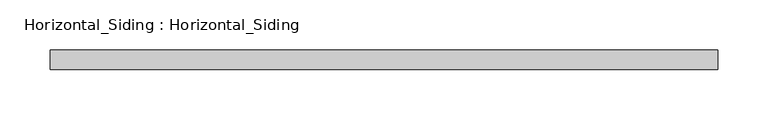
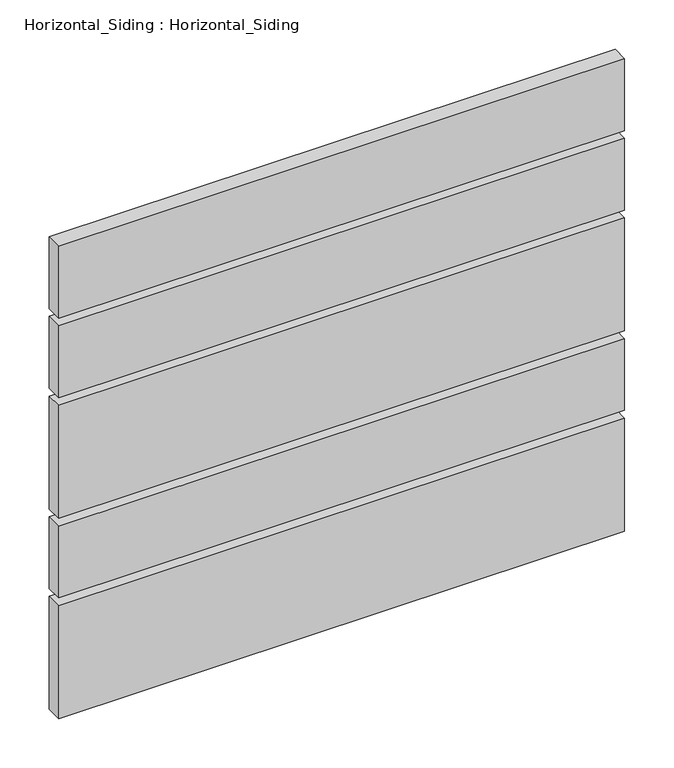
"""IFC4 building model written with IfcOpenShell, lengths in millimetres: plate geometry, Horizontal_Siding : Horizontal_Siding."""

import ifcopenshell
import ifcopenshell.guid

model = None  # the IFC model being written
_history = None  # IfcOwnerHistory: only IFC2X3 demands one
_inside = {}  # id of a spatial element -> (the spatial element, [elements in it])
_under = {}  # id of a project, library or spatial element -> (it, [spatial elements below it])
_declared = {}  # id of a project -> (the project, [libraries it declares])
_typed = {}  # id of a type object -> (the type object, [elements of that type])
_made_of = {}  # id of a material, layer set ... -> (it, [elements and type objects made of it])


def new_model(schema):
    """Start an empty IFC model of exactly this schema.

    Asked for "IFC4X3", IfcOpenShell would pick the latest addendum, in which some entities
    have other attributes; the version numbers below select the first issue.
    IFC2X3 requires an IfcOwnerHistory on every rooted entity: one is made here for all.
    """
    global model, _history
    if schema == "IFC4X3":
        model = ifcopenshell.file(schema_version=(4, 3, 0, 0))
    else:
        model = ifcopenshell.file(schema=schema)
    _inside.clear()
    _under.clear()
    _declared.clear()
    _typed.clear()
    _made_of.clear()
    _history = None
    if model.schema == "IFC2X3":
        org = make("IfcOrganization", Name="unknown")
        user = make(
            "IfcPersonAndOrganization",
            ThePerson=make("IfcPerson", FamilyName="unknown"),
            TheOrganization=org,
        )
        app = make(
            "IfcApplication",
            ApplicationDeveloper=org,
            Version="unknown",
            ApplicationFullName="unknown",
            ApplicationIdentifier="unknown",
        )
        _history = make(
            "IfcOwnerHistory",
            OwningUser=user,
            OwningApplication=app,
            ChangeAction="ADDED",
            CreationDate=0,
        )
    return model


def make(cls, **values):
    """One entity of the class cls with the attributes given. An attribute that is None is left unset."""
    return model.create_entity(
        cls, **{name: value for name, value in values.items() if value is not None}
    )


def rooted(cls, **values):
    """An entity with a GlobalId (a new one), such as an element, a storey or a relation."""
    return make(cls, GlobalId=ifcopenshell.guid.new(), OwnerHistory=_history, **values)


def si_unit(unit_type, name, prefix=None):
    """IfcSIUnit, for example si_unit("LENGTHUNIT", "METRE", prefix="MILLI")."""
    return make("IfcSIUnit", UnitType=unit_type, Prefix=prefix, Name=name)


def assignment(units):
    """IfcUnitAssignment: the units of a project."""
    return None if units is None else make("IfcUnitAssignment", Units=units)


def point(xyz):
    """IfcCartesianPoint."""
    return None if xyz is None else make("IfcCartesianPoint", Coordinates=xyz)


def direction(xyz):
    """IfcDirection."""
    return None if xyz is None else make("IfcDirection", DirectionRatios=xyz)


def frame(location, z_axis=None, x_axis=None):
    """IfcAxis2Placement3D, a coordinate frame: its origin and axes. An axis left out is left unset."""
    return make(
        "IfcAxis2Placement3D",
        Location=point(location),
        Axis=direction(z_axis),
        RefDirection=direction(x_axis),
    )


def origin():
    """The frame at (0, 0, 0) with its axes left unset."""
    return frame((0.0, 0.0, 0.0))


def place(relative_to, where):
    """IfcLocalPlacement: puts the frame where relative to a parent placement (None: the world)."""
    return make(
        "IfcLocalPlacement", PlacementRelTo=relative_to, RelativePlacement=where
    )


def context(
    kind, dimensions, precision=None, world=None, true_north=None, identifier=None
):
    """IfcGeometricRepresentationContext, for example the 3D "Model" context."""
    return make(
        "IfcGeometricRepresentationContext",
        ContextIdentifier=identifier,
        ContextType=kind,
        CoordinateSpaceDimension=dimensions,
        Precision=precision,
        WorldCoordinateSystem=world,
        TrueNorth=true_north,
    )


def project(units=None, contexts=None):
    """IfcProject with its units and contexts."""
    return rooted(
        "IfcProject",
        Name="project",
        RepresentationContexts=contexts,
        UnitsInContext=assignment(units),
    )


def spatial(cls, under=None, at=None, **own):
    """A site, building, storey or space (cls), placed at a placement, below another one or the project."""
    s = rooted(cls, ObjectPlacement=at, **own)
    if under is not None:
        _under.setdefault(under.id(), (under, []))[1].append(s)
    return s


def polyline(points):
    """IfcPolyline through the points."""
    return make("IfcPolyline", Points=[point(p) for p in points])


def outline(outer, holes=None, kind="AREA"):
    """IfcArbitraryClosedProfileDef: a profile drawn as a closed curve; with holes, ...WithVoids."""
    if holes is None:
        return make("IfcArbitraryClosedProfileDef", ProfileType=kind, OuterCurve=outer)
    return make(
        "IfcArbitraryProfileDefWithVoids",
        ProfileType=kind,
        OuterCurve=outer,
        InnerCurves=holes,
    )


def extrude(swept, where, along, depth):
    """IfcExtrudedAreaSolid: the profile swept, set in the frame where, extruded along a direction by depth."""
    return make(
        "IfcExtrudedAreaSolid",
        SweptArea=swept,
        Position=where,
        ExtrudedDirection=direction(along),
        Depth=depth,
    )


def shape(context_of_items, identifier, shape_type, items):
    """IfcShapeRepresentation: the items that make up one representation, for example the "Body"."""
    return make(
        "IfcShapeRepresentation",
        ContextOfItems=context_of_items,
        RepresentationIdentifier=identifier,
        RepresentationType=shape_type,
        Items=items,
    )


def source(mapping_origin, context_of_items, identifier, shape_type, items):
    """IfcRepresentationMap: a shape defined once, which mapped items show again and again."""
    return make(
        "IfcRepresentationMap",
        MappingOrigin=mapping_origin,
        MappedRepresentation=shape(context_of_items, identifier, shape_type, items),
    )


def transform(
    local_origin,
    x_axis=None,
    y_axis=None,
    z_axis=None,
    scale=None,
    scale2=None,
    scale3=None,
    uniform=True,
):
    """IfcCartesianTransformationOperator3D, or its non-uniform kind. x_axis, y_axis, z_axis: its Axis1, 2, 3."""
    if uniform:
        return make(
            "IfcCartesianTransformationOperator3D",
            Axis1=direction(x_axis),
            Axis2=direction(y_axis),
            LocalOrigin=point(local_origin),
            Scale=scale,
            Axis3=direction(z_axis),
        )
    return make(
        "IfcCartesianTransformationOperator3DnonUniform",
        Axis1=direction(x_axis),
        Axis2=direction(y_axis),
        LocalOrigin=point(local_origin),
        Scale=scale,
        Axis3=direction(z_axis),
        Scale2=scale2,
        Scale3=scale3,
    )


def mapped(mapping_source, mapping_target):
    """IfcMappedItem: shows the shape of a source again, moved by a transform."""
    return make(
        "IfcMappedItem", MappingSource=mapping_source, MappingTarget=mapping_target
    )


def made_of(thing, what):
    """Note that an element or type object is made of a material, layer set ...; save() writes the relation."""
    if what is not None:
        _made_of.setdefault(what.id(), (what, []))[1].append(thing)
    return thing


def element(
    cls,
    number,
    at=None,
    inside=None,
    cuts=None,
    type_object=None,
    material=None,
    context=None,
    identifier="Body",
    shape_type=None,
    held_by="IfcProductDefinitionShape",
    body=None,
    shapes=None,
    **own,
):
    """One element of the class cls, such as IfcWall. Its Tag is "e" and its number.

    at: its placement. inside: the storey or other place that contains it. cuts: it is an
    opening in that element (IfcRelVoidsElement). A single representation is given by context,
    identifier, shape_type and body (its items); several are given by shapes. held_by: the class
    of the entity that holds the representations. save() writes the other relations.
    """
    e = rooted(cls, Tag="e%d" % number, ObjectPlacement=at, **own)
    if body is not None:
        shapes = [shape(context, identifier, shape_type, body)]
    if shapes is not None:
        e.Representation = make(held_by, Representations=shapes)
    if inside is not None:
        _inside.setdefault(inside.id(), (inside, []))[1].append(e)
    if cuts is not None:
        rooted(
            "IfcRelVoidsElement", RelatingBuildingElement=cuts, RelatedOpeningElement=e
        )
    if type_object is not None:
        _typed.setdefault(type_object.id(), (type_object, []))[1].append(e)
    return made_of(e, material)


def aggregate(whole, parts):
    """IfcRelAggregates: a whole, such as a stair, and the parts it consists of."""
    return rooted("IfcRelAggregates", RelatingObject=whole, RelatedObjects=parts)


def save(model, path):
    """Write the relations noted so far, then the file.

    IfcRelAggregates (storeys below a building ...), IfcRelContainedInSpatialStructure (elements
    in a storey), IfcRelDefinesByType, IfcRelAssociatesMaterial and IfcRelDeclares: one each for
    every whole, place, type object, material and project.
    """
    for whole, parts in _under.values():
        aggregate(whole, parts)
    for where, things in _inside.values():
        rooted(
            "IfcRelContainedInSpatialStructure",
            RelatedElements=things,
            RelatingStructure=where,
        )
    for kind, things in _typed.values():
        rooted("IfcRelDefinesByType", RelatedObjects=things, RelatingType=kind)
    for what, things in _made_of.values():
        rooted("IfcRelAssociatesMaterial", RelatedObjects=things, RelatingMaterial=what)
    for by, libraries in _declared.values():
        rooted("IfcRelDeclares", RelatingContext=by, RelatedDefinitions=libraries)
    model.write(path)


def horizontal_siding_horizontal_siding_c9112cef(model_context):
    return source(origin(), model_context, "Body", "SweptSolid", [
        extrude(outline(polyline([(331.1333097, -19.05), (-331.1333097, -19.05), (-331.1333097, 0.0), (331.1333097, 0.0), (331.1333097, -19.05)])), frame((0.0, 0.0, 9.525), z_axis=(0.0, 0.0, 1.0), x_axis=(1.0, 0.0, 0.0)), (0.0, 0.0, 1.0), 139.7),
        extrude(outline(polyline([(331.1333097, -19.05), (-331.1333097, -19.05), (-331.1333097, 0.0), (331.1333097, 0.0), (331.1333097, -19.05)])), frame((0.0, 0.0, 158.75), z_axis=(0.0, 0.0, 1.0), x_axis=(1.0, 0.0, 0.0)), (0.0, 0.0, 1.0), 88.9),
        extrude(outline(polyline([(331.1333097, -19.05), (-331.1333097, -19.05), (-331.1333097, 0.0), (331.1333097, 0.0), (331.1333097, -19.05)])), frame((0.0, 0.0, 257.175), z_axis=(0.0, 0.0, 1.0), x_axis=(1.0, 0.0, 0.0)), (0.0, 0.0, 1.0), 139.7),
        extrude(outline(polyline([(331.1333097, -19.05), (-331.1333097, -19.05), (-331.1333097, 0.0), (331.1333097, 0.0), (331.1333097, -19.05)])), frame((0.0, 0.0, 406.4), z_axis=(0.0, 0.0, 1.0), x_axis=(1.0, 0.0, 0.0)), (0.0, 0.0, 1.0), 88.9),
        extrude(outline(polyline([(331.1333097, -19.05), (-331.1333097, -19.05), (-331.1333097, 0.0), (331.1333097, 0.0), (331.1333097, -19.05)])), frame((0.0, 0.0, 504.825), z_axis=(0.0, 0.0, 1.0), x_axis=(1.0, 0.0, 0.0)), (0.0, 0.0, 1.0), 88.9),
    ])


if __name__ == "__main__":
    model = new_model("IFC4")
    model_context = context("Model", 3, world=origin())
    ifc_project = project(units=[si_unit("LENGTHUNIT", "METRE", prefix="MILLI")], contexts=[model_context])
    site = spatial("IfcSite", under=ifc_project)
    building = spatial("IfcBuilding", under=site)
    placement = place(None, origin())
    horizontal_siding_horizontal_siding_shape = horizontal_siding_horizontal_siding_c9112cef(model_context)
    element("IfcPlate", 1, ObjectType="Horizontal_Siding : Horizontal_Siding", at=placement, inside=building, context=model_context, shape_type="MappedRepresentation", body=[
        mapped(horizontal_siding_horizontal_siding_shape, transform((0.0, 0.0, 0.0), x_axis=(1.0, 0.0, 0.0), y_axis=(0.0, 1.0, 0.0), z_axis=(0.0, 0.0, 1.0))),
    ])
    save(model, "model.ifc")

# Revit data of these elements
# Type "Horizontal_Siding : Horizontal_Siding"
#   Analytic Construction = "<None>"
#   extend = 0' - 2 3/4"
#   Width_2 = 0' - 3 1/2"
#   Width_1 = 0' - 5 1/2"
#   Gap = 0' - 0 3/8"
#   Plank Material = SLOTTED WOOD FENCE (THERMALLY MODIFIED WOOD: ARBOR WOOD)\n(EXTERIOR STAIN : PENOFIN VERDE EXT. STAIN - COLOR: CEDAR)
# Element 1 (IfcPlate, "Horizontal_Siding : Horizontal_Siding")
#   Materials on its faces: "SLOTTED WOOD FENCE (THERMALLY MODIFIED WOOD: ARBOR WOOD)\n(EXTERIOR STAIN : PENOFIN VERDE EXT. STAIN - COLOR: CEDAR)"
# Materials
#   "SLOTTED WOOD FENCE (THERMALLY MODIFIED WOOD: ARBOR WOOD)\n(EXTERIOR STAIN : PENOFIN VERDE EXT. STAIN - COLOR: CEDAR)": class "Wood", colour RGB 164 134 123, transparency 0, Description = "Pinus Echinata", Cost = 0
